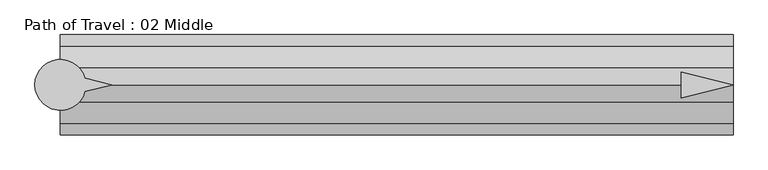
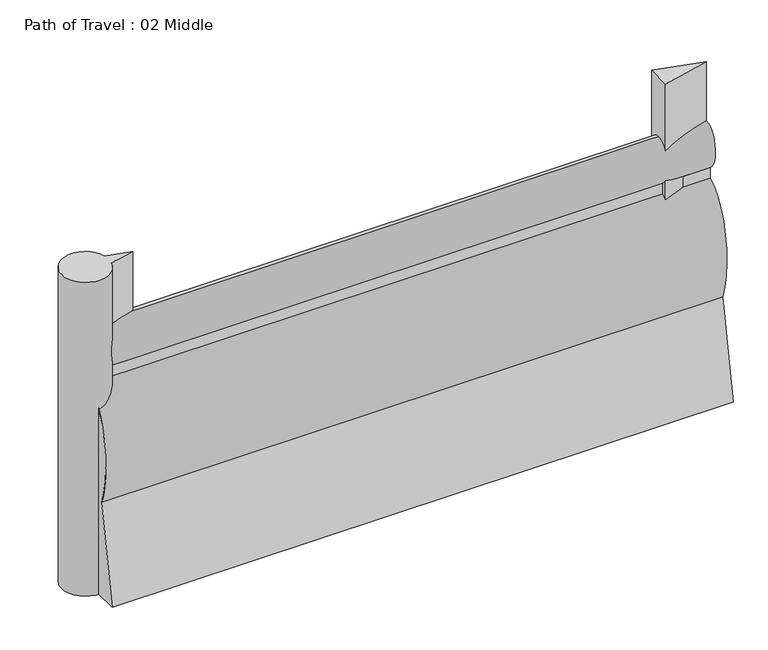
"""IFC4 building model written with IfcOpenShell, lengths in millimetres: proxy geometry, Path of Travel : 02 Middle."""

from ifc_helpers import new_model, si_unit, point, frame, frame_2d, origin, origin_with_axes, place, context, project, spatial, polyline, circle_curve, ellipse_curve, trimmed, segment, composite_curve, outline, extrude, source, transform, mapped, element, save
from ifc_brep_helpers import plane_surface, extruded_surface, advanced_brep


def path_of_travel_02_middle_9a7ea904(model_context):
    return source(origin(), model_context, "Body", "SolidModel", [
        advanced_brep(
        [(227.5554837, 0.0, 1727.2), (227.5554837, 42.9018657, 1436.6534209), (227.5554837, 42.9018657, 1363.4763406), (227.5554837, 184.1186263, 643.4144547), (227.5554837, 297.5699544, 0.0), (227.5554837, 145.6574193, 0.0), (227.5554837, 0.0, 584.2), (227.5554837, -145.6574193, 0.0), (227.5554837, -297.5699544, 0.0), (227.5554837, -184.1186263, 643.4144547), (227.5554837, -42.9018657, 1363.4763406), (227.5554837, -42.9018657, 1436.6534209), (4212.0051488, 0.0, 1727.2), (4212.0051488, -42.9018657, 1436.6534209), (4212.0051488, -42.9018657, 1363.4763406), (4212.0051488, -184.1186263, 643.4144547), (4212.0051488, -297.5699544, 0.0), (4212.0051488, -145.6574193, 0.0), (4212.0051488, 0.0, 584.2), (4212.0051488, 145.6574193, 0.0), (4212.0051488, 297.5699544, 0.0), (4212.0051488, 184.1186263, 643.4144547), (4212.0051488, 42.9018657, 1363.4763406), (4212.0051488, 42.9018657, 1436.6534209)],
        [
            (0, 1, ellipse_curve(frame((227.5554837, 0.0, 1574.8), z_axis=(-1.0, 0.0, 0.0), x_axis=(0.0, 0.0, 1.0)), 152.4, 101.6)),
            (1, 2),
            (2, 3, ellipse_curve(frame((227.5554837, 0.0, 914.4), z_axis=(-1.0, 0.0, 0.0), x_axis=(0.0, 0.0, -1.0)), 457.2, 228.6)),
            (3, 4),
            (4, 5),
            (5, 6),
            (6, 7),
            (7, 8),
            (8, 9),
            (9, 10, ellipse_curve(frame((227.5554837, 0.0, 914.4), z_axis=(-1.0, 0.0, 0.0), x_axis=(0.0, 0.0, -1.0)), 457.2, 228.6)),
            (10, 11),
            (11, 0, ellipse_curve(frame((227.5554837, 0.0, 1574.8), z_axis=(-1.0, 0.0, 0.0), x_axis=(0.0, 0.0, 1.0)), 152.4, 101.6)),
            (12, 13, ellipse_curve(frame((4212.0051488, 0.0, 1574.8), z_axis=(1.0, 0.0, 0.0), x_axis=(0.0, 0.0, 1.0)), 152.4, 101.6)),
            (13, 14),
            (14, 15, ellipse_curve(frame((4212.0051488, 0.0, 914.4), z_axis=(1.0, 0.0, 0.0), x_axis=(0.0, 0.0, -1.0)), 457.2, 228.6)),
            (15, 16),
            (16, 17),
            (17, 18),
            (18, 19),
            (19, 20),
            (20, 21),
            (21, 22, ellipse_curve(frame((4212.0051488, 0.0, 914.4), z_axis=(1.0, 0.0, 0.0), x_axis=(0.0, 0.0, -1.0)), 457.2, 228.6)),
            (22, 23),
            (23, 12, ellipse_curve(frame((4212.0051488, 0.0, 1574.8), z_axis=(1.0, 0.0, 0.0), x_axis=(0.0, 0.0, 1.0)), 152.4, 101.6)),
            (0, 12),
            (23, 1),
            (22, 2),
            (21, 3),
            (20, 4),
            (19, 5),
            (18, 6),
            (17, 7),
            (16, 8),
            (15, 9),
            (14, 10),
            (13, 11),
        ],
        [
            plane_surface(frame((227.5554837, 0.0, 0.0), z_axis=(-1.0, 0.0, 0.0), x_axis=(0.0, 0.0, 1.0))),
            plane_surface(frame((4212.0051488, 0.0, 0.0), z_axis=(1.0, 0.0, 0.0), x_axis=(0.0, 0.0, 1.0))),
            extruded_surface(trimmed(ellipse_curve(frame((4212.0051488, 0.0, 1574.8), z_axis=(-1.0, 0.0, 0.0), x_axis=(0.0, 0.0, 1.0)), 152.4, 101.6), [point((4212.0051488, 0.0, 1727.2))], [point((4212.0051488, 42.9018657, 1436.6534209))], True, "CARTESIAN"), (-3984.4496651, 0.0, 0.0), 3984.4496651),
            plane_surface(frame((227.5554837, 42.9018657, 1436.6534209), z_axis=(0.0, 1.0, 0.0), x_axis=(1.0, 0.0, 0.0))),
            extruded_surface(trimmed(ellipse_curve(frame((4212.0051488, 0.0, 914.4), z_axis=(-1.0, 0.0, 0.0), x_axis=(0.0, 0.0, -1.0)), 457.2, 228.6), [point((4212.0051488, 42.9018657, 1363.4763406))], [point((4212.0051488, 184.1186263, 643.4144547))], True, "CARTESIAN"), (-3984.4496651, 0.0, 0.0), 3984.4496651),
            plane_surface(frame((227.5554837, 184.1186263, 643.4144547), z_axis=(0.0, 0.9848077530122078, 0.1736481776669322), x_axis=(1.0, 0.0, 0.0))),
            plane_surface(frame((227.5554837, 297.5699544, 0.0), z_axis=(0.0, 0.0, -1.0), x_axis=(1.0, 0.0, 0.0))),
            plane_surface(frame((227.5554837, 145.6574193, 0.0), z_axis=(0.0, -0.9702957262760199, -0.2419218955995739), x_axis=(1.0, 0.0, 0.0))),
            plane_surface(frame((227.5554837, 0.0, 584.2), z_axis=(0.0, 0.9702957262759961, -0.24192189559966923), x_axis=(1.0, 0.0, 0.0))),
            plane_surface(frame((227.5554837, -145.6574193, 0.0), z_axis=(0.0, 0.0, -1.0), x_axis=(1.0, 0.0, 0.0))),
            plane_surface(frame((227.5554837, -297.5699544, 0.0), z_axis=(0.0, -0.984807753012208, 0.17364817766693066), x_axis=(1.0, 0.0, 0.0))),
            extruded_surface(trimmed(ellipse_curve(frame((4212.0051488, 0.0, 914.4), z_axis=(-1.0, 0.0, 0.0), x_axis=(0.0, 0.0, -1.0)), 457.2, 228.6), [point((4212.0051488, -184.1186263, 643.4144547))], [point((4212.0051488, -42.9018657, 1363.4763406))], True, "CARTESIAN"), (-3984.4496651, 0.0, 0.0), 3984.4496651),
            plane_surface(frame((227.5554837, -42.9018657, 1363.4763406), z_axis=(0.0, -1.0, 0.0), x_axis=(1.0, 0.0, 0.0))),
            extruded_surface(trimmed(ellipse_curve(frame((4212.0051488, 0.0, 1574.8), z_axis=(-1.0, 0.0, 0.0), x_axis=(0.0, 0.0, 1.0)), 152.4, 101.6), [point((4212.0051488, -42.9018657, 1436.6534209))], [point((4212.0051488, 0.0, 1727.2))], True, "CARTESIAN"), (-3984.4496651, 0.0, 0.0), 3984.4496651),
        ],
        [
            (0, [[1, 2, 3, 4, 5, 6, 7, 8, 9, 10, 11, 12]]),
            (1, [[13, 14, 15, 16, 17, 18, 19, 20, 21, 22, 23, 24]]),
            (2, [[-1, 25, -24, 26]]),
            (3, [[-2, -26, -23, 27]]),
            (4, [[-3, -27, -22, 28]]),
            (5, [[-4, -28, -21, 29]]),
            (6, [[-5, -29, -20, 30]]),
            (7, [[-6, -30, -19, 31]]),
            (8, [[-7, -31, -18, 32]]),
            (9, [[-8, -32, -17, 33]]),
            (10, [[-9, -33, -16, 34]]),
            (11, [[-10, -34, -15, 35]]),
            (12, [[-11, -35, -14, 36]]),
            (13, [[-12, -36, -13, -25]]),
        ],
    ),
        extrude(outline(polyline([(3906.0000022, 76.2006338), (4212.0051488, 0.0), (3906.0000022, -76.2006338), (3906.0000022, 76.2006338)])), origin_with_axes(), (0.0, 0.0, 1.0), 2129.5973753),
        extrude(outline(composite_curve([segment(polyline([(372.7837828, 39.4440225), (531.182385, 0.0), (372.7837828, -39.4440225)]), True, "CONTINUOUS"), segment(trimmed(circle_curve(frame_2d((227.2200886, 0.0)), 150.8131956), [point((372.7837828, -39.4440225))], [point((372.7837828, 39.4440225))], False, "CARTESIAN"), True, "CONTINUOUS")], self_intersect=False)), origin_with_axes(), (0.0, 0.0, 1.0), 2129.5973753),
    ])


if __name__ == "__main__":
    model = new_model("IFC4")
    model_context = context("Model", 3, world=origin())
    ifc_project = project(units=[si_unit("LENGTHUNIT", "METRE", prefix="MILLI")], contexts=[model_context])
    site = spatial("IfcSite", under=ifc_project)
    building = spatial("IfcBuilding", under=site)
    placement = place(None, origin())
    path_of_travel_02_middle_shape = path_of_travel_02_middle_9a7ea904(model_context)
    element("IfcBuildingElementProxy", 1, Name="Path of Travel : 02 Middle", ObjectType="Path of Travel : 02 Middle", at=placement, inside=building, context=model_context, shape_type="MappedRepresentation", body=[
        mapped(path_of_travel_02_middle_shape, transform((0.0, 0.0, 0.0), x_axis=(1.0, 0.0, 0.0), y_axis=(0.0, 1.0, 0.0), z_axis=(0.0, 0.0, 1.0))),
    ])
    save(model, "model.ifc")

# Revit data of these elements
# Type "Path of Travel : 02 Middle"
#   Path of Egress [instance default] = 4' - 0"
#   built-in parameter 1001306 [instance default] = 4 (stored number, unit not read)
#   Dot at Start = no
#   Arrow in Middle = yes
#   Arrow at End = no
#   Egress Path = none
# Element 1 (IfcBuildingElementProxy, "Path of Travel : 02 Middle")
#   Path of Egress = 13' - 0.8681"
#   built-in parameter 1001306 = 13.0723 (stored number, unit not read)
#   Materials on its faces: "Egress Path Solid", "solid"
# Materials
#   "Egress Path Solid": class "Unassigned", colour RGB 255 128 64, transparency 0.75, Comments = "Rendering appearance not upgraded "
#   "solid": class "Generic", colour RGB 120 120 120, transparency 0, Cost = 0
